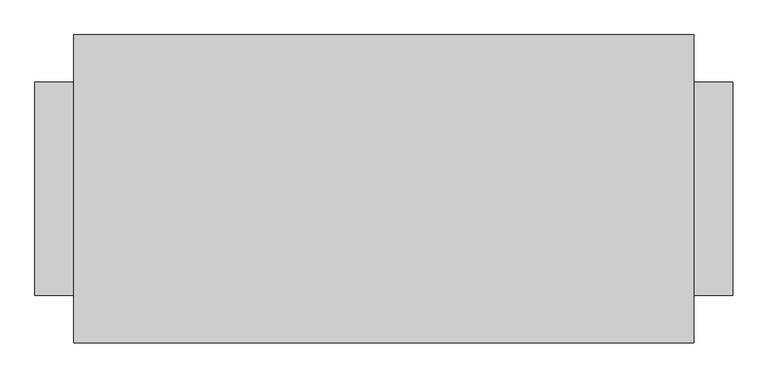
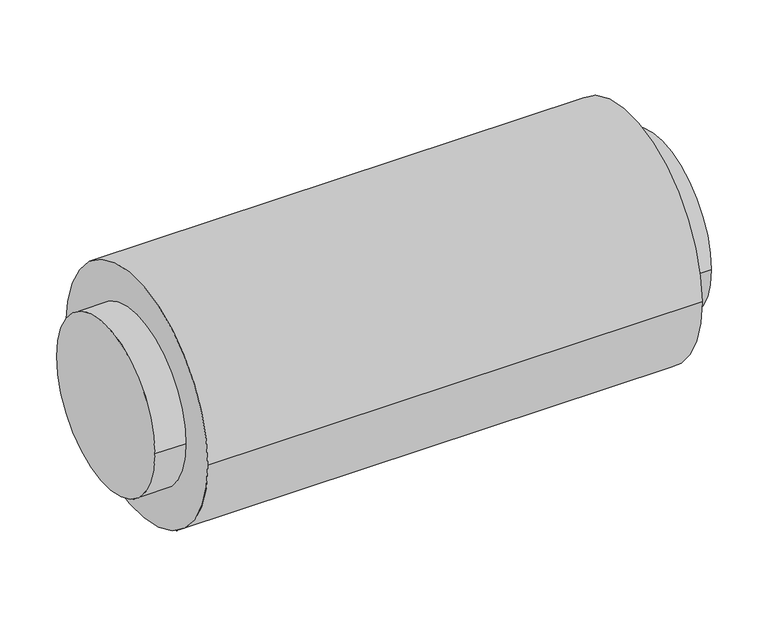
"""IFC4 building model written with IfcOpenShell, lengths in millimetres: proxy geometry, Шумоглушитель DRQ : Шумоглушитель DRQ 315/9."""

from ifc_helpers import new_model, si_unit, point, frame, origin, origin_2d, place, context, project, spatial, circle_curve, trimmed, segment, composite_curve, outline, extrude, source, transform, mapped, element, save


def mechanical_equipment_3d923659(model_context):
    return source(origin(), model_context, "Body", "SweptSolid", [
        extrude(outline(composite_curve([segment(trimmed(circle_curve(origin_2d(), 157.5), [point((-157.5, 0.0))], [point((157.5, 0.0))], False, "CARTESIAN"), True, "CONTINUOUS"), segment(trimmed(circle_curve(origin_2d(), 157.5), [point((157.5, 0.0))], [point((-157.5, 0.0))], False, "CARTESIAN"), True, "CONTINUOUS")], self_intersect=False)), frame((-515.0, 0.0, 0.0), z_axis=(1.0, 0.0, 0.0), x_axis=(0.0, 1.0, 0.0)), (0.0, 0.0, 1.0), 57.5),
        extrude(outline(composite_curve([segment(trimmed(circle_curve(origin_2d(), 227.5), [point((-227.5, 0.0))], [point((227.5, 0.0))], False, "CARTESIAN"), True, "CONTINUOUS"), segment(trimmed(circle_curve(origin_2d(), 227.5), [point((227.5, 0.0))], [point((-227.5, 0.0))], False, "CARTESIAN"), True, "CONTINUOUS")], self_intersect=False)), frame((-457.5, 0.0, 0.0), z_axis=(1.0, 0.0, 0.0), x_axis=(0.0, 1.0, 0.0)), (0.0, 0.0, 1.0), 915.0),
        extrude(outline(composite_curve([segment(trimmed(circle_curve(origin_2d(), 157.5), [point((-157.5, 0.0))], [point((157.5, 0.0))], False, "CARTESIAN"), True, "CONTINUOUS"), segment(trimmed(circle_curve(origin_2d(), 157.5), [point((157.5, 0.0))], [point((-157.5, 0.0))], False, "CARTESIAN"), True, "CONTINUOUS")], self_intersect=False)), frame((457.5, 0.0, 0.0), z_axis=(1.0, 0.0, 0.0), x_axis=(0.0, 1.0, 0.0)), (0.0, 0.0, 1.0), 57.5),
    ])


if __name__ == "__main__":
    model = new_model("IFC4")
    model_context = context("Model", 3, world=origin())
    ifc_project = project(units=[si_unit("LENGTHUNIT", "METRE", prefix="MILLI")], contexts=[model_context])
    site = spatial("IfcSite", under=ifc_project)
    building = spatial("IfcBuilding", under=site)
    placement = place(None, origin())
    mechanical_equipment_shape = mechanical_equipment_3d923659(model_context)
    element("IfcBuildingElementProxy", 1, Name="Шумоглушитель DRQ : Шумоглушитель DRQ 315/9", ObjectType="Шумоглушитель DRQ : Шумоглушитель DRQ 315/9", at=placement, inside=building, context=model_context, shape_type="MappedRepresentation", body=[
        mapped(mechanical_equipment_shape, transform((0.0, 0.0, 0.0), x_axis=(1.0, 0.0, 0.0), y_axis=(0.0, 1.0, 0.0), z_axis=(0.0, 0.0, 1.0))),
    ])
    save(model, "model.ifc")

# Revit data of these elements
# Type "Шумоглушитель DRQ : Шумоглушитель DRQ 315/9"
#   Manufacturer = "WAER"
#   ADSK_Система_Имя [instance default] = ""
#   ADSK_Наименование краткое = "DRQ 315/9"
#   ADSK_Наименование [instance default] = "Шумоглушитель DRQ 315/9"
#   ADSK_Масса_Текст = "14"
#   ADSK_Марка = "DRQ 315/9"
#   ADSK_Код изделия = "Шумоглушитель DRQ 315/9"
#   ADSK_Завод-изготовитель = "WAER"
#   ADSK_Единица измерения = "шт."
#   ADSK_URL страницы изделия = "https://waer-air.com/shumoglushiteli-drq/"
#   ADSK_URL документации изделия = "https://waer-air.com/data/uploads/download/channel-equipment-waer.pdf"
#   ADSK_Размер_Длина_А = 915 mm
#   ADSK_Размер_Диаметр_Б = 455 mm
#   Cost = 1
#   ADSK_Расход воздуха = 300 m³/h
#   ADSK_Размер_Длина_В = 1030 mm
#   ADSK_Размер_Диаметр_Д = 315 mm
#   ADSK_Потеря давления воздуха = 0.0 Pa
#   ADSK_Масса = 14
#   ADSK_Количество [instance default] = 1
#   Default Elevation = 0
#   URL = ""
